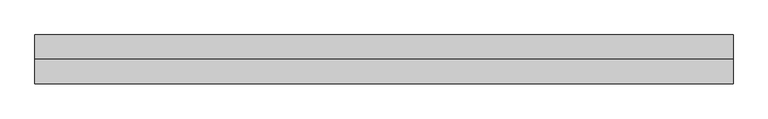
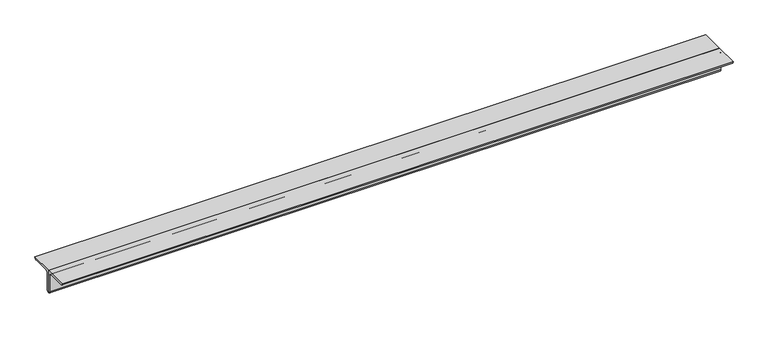
"""IFC4 building model written with IfcOpenShell, lengths in millimetres: member geometry, 0123_Steel Framing_2Ls-KSD3502 : H_SB_AR_S03_2Ls-130x130x12_HBR1."""

import ifcopenshell
import ifcopenshell.guid

model = None  # the IFC model being written
_history = None  # IfcOwnerHistory: only IFC2X3 demands one
_inside = {}  # id of a spatial element -> (the spatial element, [elements in it])
_under = {}  # id of a project, library or spatial element -> (it, [spatial elements below it])
_declared = {}  # id of a project -> (the project, [libraries it declares])
_typed = {}  # id of a type object -> (the type object, [elements of that type])
_made_of = {}  # id of a material, layer set ... -> (it, [elements and type objects made of it])


def new_model(schema):
    """Start an empty IFC model of exactly this schema.

    Asked for "IFC4X3", IfcOpenShell would pick the latest addendum, in which some entities
    have other attributes; the version numbers below select the first issue.
    IFC2X3 requires an IfcOwnerHistory on every rooted entity: one is made here for all.
    """
    global model, _history
    if schema == "IFC4X3":
        model = ifcopenshell.file(schema_version=(4, 3, 0, 0))
    else:
        model = ifcopenshell.file(schema=schema)
    _inside.clear()
    _under.clear()
    _declared.clear()
    _typed.clear()
    _made_of.clear()
    _history = None
    if model.schema == "IFC2X3":
        org = make("IfcOrganization", Name="unknown")
        user = make(
            "IfcPersonAndOrganization",
            ThePerson=make("IfcPerson", FamilyName="unknown"),
            TheOrganization=org,
        )
        app = make(
            "IfcApplication",
            ApplicationDeveloper=org,
            Version="unknown",
            ApplicationFullName="unknown",
            ApplicationIdentifier="unknown",
        )
        _history = make(
            "IfcOwnerHistory",
            OwningUser=user,
            OwningApplication=app,
            ChangeAction="ADDED",
            CreationDate=0,
        )
    return model


def make(cls, **values):
    """One entity of the class cls with the attributes given. An attribute that is None is left unset."""
    return model.create_entity(
        cls, **{name: value for name, value in values.items() if value is not None}
    )


def rooted(cls, **values):
    """An entity with a GlobalId (a new one), such as an element, a storey or a relation."""
    return make(cls, GlobalId=ifcopenshell.guid.new(), OwnerHistory=_history, **values)


def si_unit(unit_type, name, prefix=None):
    """IfcSIUnit, for example si_unit("LENGTHUNIT", "METRE", prefix="MILLI")."""
    return make("IfcSIUnit", UnitType=unit_type, Prefix=prefix, Name=name)


def assignment(units):
    """IfcUnitAssignment: the units of a project."""
    return None if units is None else make("IfcUnitAssignment", Units=units)


def point(xyz):
    """IfcCartesianPoint."""
    return None if xyz is None else make("IfcCartesianPoint", Coordinates=xyz)


def direction(xyz):
    """IfcDirection."""
    return None if xyz is None else make("IfcDirection", DirectionRatios=xyz)


def frame(location, z_axis=None, x_axis=None):
    """IfcAxis2Placement3D, a coordinate frame: its origin and axes. An axis left out is left unset."""
    return make(
        "IfcAxis2Placement3D",
        Location=point(location),
        Axis=direction(z_axis),
        RefDirection=direction(x_axis),
    )


def frame_2d(location, x_axis=None):
    """IfcAxis2Placement2D, a coordinate frame in the plane: its origin and x axis."""
    return make(
        "IfcAxis2Placement2D", Location=point(location), RefDirection=direction(x_axis)
    )


def origin():
    """The frame at (0, 0, 0) with its axes left unset."""
    return frame((0.0, 0.0, 0.0))


def place(relative_to, where):
    """IfcLocalPlacement: puts the frame where relative to a parent placement (None: the world)."""
    return make(
        "IfcLocalPlacement", PlacementRelTo=relative_to, RelativePlacement=where
    )


def context(
    kind, dimensions, precision=None, world=None, true_north=None, identifier=None
):
    """IfcGeometricRepresentationContext, for example the 3D "Model" context."""
    return make(
        "IfcGeometricRepresentationContext",
        ContextIdentifier=identifier,
        ContextType=kind,
        CoordinateSpaceDimension=dimensions,
        Precision=precision,
        WorldCoordinateSystem=world,
        TrueNorth=true_north,
    )


def project(units=None, contexts=None):
    """IfcProject with its units and contexts."""
    return rooted(
        "IfcProject",
        Name="project",
        RepresentationContexts=contexts,
        UnitsInContext=assignment(units),
    )


def spatial(cls, under=None, at=None, **own):
    """A site, building, storey or space (cls), placed at a placement, below another one or the project."""
    s = rooted(cls, ObjectPlacement=at, **own)
    if under is not None:
        _under.setdefault(under.id(), (under, []))[1].append(s)
    return s


def polyline(points):
    """IfcPolyline through the points."""
    return make("IfcPolyline", Points=[point(p) for p in points])


def circle_curve(where, radius):
    """IfcCircle in the frame where."""
    return make("IfcCircle", Position=where, Radius=radius)


def trimmed(basis, trim1, trim2, sense, master):
    """IfcTrimmedCurve: the piece of a basis curve between two trims."""
    return make(
        "IfcTrimmedCurve",
        BasisCurve=basis,
        Trim1=trim1,
        Trim2=trim2,
        SenseAgreement=sense,
        MasterRepresentation=master,
    )


def segment(curve, same_sense, transition):
    """IfcCompositeCurveSegment."""
    return make(
        "IfcCompositeCurveSegment",
        Transition=transition,
        SameSense=same_sense,
        ParentCurve=curve,
    )


def composite_curve(segments, self_intersect=None):
    """IfcCompositeCurve: segments joined end to end."""
    return make("IfcCompositeCurve", Segments=segments, SelfIntersect=self_intersect)


def outline(outer, holes=None, kind="AREA"):
    """IfcArbitraryClosedProfileDef: a profile drawn as a closed curve; with holes, ...WithVoids."""
    if holes is None:
        return make("IfcArbitraryClosedProfileDef", ProfileType=kind, OuterCurve=outer)
    return make(
        "IfcArbitraryProfileDefWithVoids",
        ProfileType=kind,
        OuterCurve=outer,
        InnerCurves=holes,
    )


def extrude(swept, where, along, depth):
    """IfcExtrudedAreaSolid: the profile swept, set in the frame where, extruded along a direction by depth."""
    return make(
        "IfcExtrudedAreaSolid",
        SweptArea=swept,
        Position=where,
        ExtrudedDirection=direction(along),
        Depth=depth,
    )


def shape(context_of_items, identifier, shape_type, items):
    """IfcShapeRepresentation: the items that make up one representation, for example the "Body"."""
    return make(
        "IfcShapeRepresentation",
        ContextOfItems=context_of_items,
        RepresentationIdentifier=identifier,
        RepresentationType=shape_type,
        Items=items,
    )


def source(mapping_origin, context_of_items, identifier, shape_type, items):
    """IfcRepresentationMap: a shape defined once, which mapped items show again and again."""
    return make(
        "IfcRepresentationMap",
        MappingOrigin=mapping_origin,
        MappedRepresentation=shape(context_of_items, identifier, shape_type, items),
    )


def transform(
    local_origin,
    x_axis=None,
    y_axis=None,
    z_axis=None,
    scale=None,
    scale2=None,
    scale3=None,
    uniform=True,
):
    """IfcCartesianTransformationOperator3D, or its non-uniform kind. x_axis, y_axis, z_axis: its Axis1, 2, 3."""
    if uniform:
        return make(
            "IfcCartesianTransformationOperator3D",
            Axis1=direction(x_axis),
            Axis2=direction(y_axis),
            LocalOrigin=point(local_origin),
            Scale=scale,
            Axis3=direction(z_axis),
        )
    return make(
        "IfcCartesianTransformationOperator3DnonUniform",
        Axis1=direction(x_axis),
        Axis2=direction(y_axis),
        LocalOrigin=point(local_origin),
        Scale=scale,
        Axis3=direction(z_axis),
        Scale2=scale2,
        Scale3=scale3,
    )


def mapped(mapping_source, mapping_target):
    """IfcMappedItem: shows the shape of a source again, moved by a transform."""
    return make(
        "IfcMappedItem", MappingSource=mapping_source, MappingTarget=mapping_target
    )


def made_of(thing, what):
    """Note that an element or type object is made of a material, layer set ...; save() writes the relation."""
    if what is not None:
        _made_of.setdefault(what.id(), (what, []))[1].append(thing)
    return thing


def element(
    cls,
    number,
    at=None,
    inside=None,
    cuts=None,
    type_object=None,
    material=None,
    context=None,
    identifier="Body",
    shape_type=None,
    held_by="IfcProductDefinitionShape",
    body=None,
    shapes=None,
    **own,
):
    """One element of the class cls, such as IfcWall. Its Tag is "e" and its number.

    at: its placement. inside: the storey or other place that contains it. cuts: it is an
    opening in that element (IfcRelVoidsElement). A single representation is given by context,
    identifier, shape_type and body (its items); several are given by shapes. held_by: the class
    of the entity that holds the representations. save() writes the other relations.
    """
    e = rooted(cls, Tag="e%d" % number, ObjectPlacement=at, **own)
    if body is not None:
        shapes = [shape(context, identifier, shape_type, body)]
    if shapes is not None:
        e.Representation = make(held_by, Representations=shapes)
    if inside is not None:
        _inside.setdefault(inside.id(), (inside, []))[1].append(e)
    if cuts is not None:
        rooted(
            "IfcRelVoidsElement", RelatingBuildingElement=cuts, RelatedOpeningElement=e
        )
    if type_object is not None:
        _typed.setdefault(type_object.id(), (type_object, []))[1].append(e)
    return made_of(e, material)


def aggregate(whole, parts):
    """IfcRelAggregates: a whole, such as a stair, and the parts it consists of."""
    return rooted("IfcRelAggregates", RelatingObject=whole, RelatedObjects=parts)


def save(model, path):
    """Write the relations noted so far, then the file.

    IfcRelAggregates (storeys below a building ...), IfcRelContainedInSpatialStructure (elements
    in a storey), IfcRelDefinesByType, IfcRelAssociatesMaterial and IfcRelDeclares: one each for
    every whole, place, type object, material and project.
    """
    for whole, parts in _under.values():
        aggregate(whole, parts)
    for where, things in _inside.values():
        rooted(
            "IfcRelContainedInSpatialStructure",
            RelatedElements=things,
            RelatingStructure=where,
        )
    for kind, things in _typed.values():
        rooted("IfcRelDefinesByType", RelatedObjects=things, RelatingType=kind)
    for what, things in _made_of.values():
        rooted("IfcRelAssociatesMaterial", RelatedObjects=things, RelatingMaterial=what)
    for by, libraries in _declared.values():
        rooted("IfcRelDeclares", RelatingContext=by, RelatedDefinitions=libraries)
    model.write(path)


def member_2dd2a1f8(model_context):
    return source(origin(), model_context, "Body", "SweptSolid", [
        extrude(outline(composite_curve([segment(polyline([(0.0, 36.4), (0.0, -93.6)]), True, "CONTINUOUS"), segment(trimmed(circle_curve(frame_2d((0.0, -81.6)), 12.0), [point((0.0, -93.6))], [point((-12.0, -81.6))], False, "CARTESIAN"), True, "CONTINUOUS"), segment(polyline([(-12.0, -81.6), (-12.0, 12.4)]), True, "CONTINUOUS"), segment(trimmed(circle_curve(frame_2d((-24.0, 12.4)), 12.0), [point((-12.0, 12.4))], [point((-24.0, 24.4))], True, "CARTESIAN"), True, "CONTINUOUS"), segment(polyline([(-24.0, 24.4), (-118.0, 24.4)]), True, "CONTINUOUS"), segment(trimmed(circle_curve(frame_2d((-118.0, 36.4)), 12.0), [point((-118.0, 24.4))], [point((-130.0, 36.4))], False, "CARTESIAN"), True, "CONTINUOUS"), segment(polyline([(-130.0, 36.4), (0.0, 36.4)]), True, "CONTINUOUS")], self_intersect=False)), frame((-1830.7666695, 0.0, 0.0), z_axis=(1.0, 0.0, 0.0), x_axis=(0.0, 1.0, 0.0)), (0.0, 0.0, 1.0), 3701.6272171),
        extrude(outline(composite_curve([segment(polyline([(0.0, 36.4), (130.0, 36.4)]), True, "CONTINUOUS"), segment(trimmed(circle_curve(frame_2d((118.0, 36.4)), 12.0), [point((130.0, 36.4))], [point((118.0, 24.4))], False, "CARTESIAN"), True, "CONTINUOUS"), segment(polyline([(118.0, 24.4), (24.0, 24.4)]), True, "CONTINUOUS"), segment(trimmed(circle_curve(frame_2d((24.0, 12.4)), 12.0), [point((24.0, 24.4))], [point((12.0, 12.4))], True, "CARTESIAN"), True, "CONTINUOUS"), segment(polyline([(12.0, 12.4), (12.0, -81.6)]), True, "CONTINUOUS"), segment(trimmed(circle_curve(frame_2d((0.0, -81.6)), 12.0), [point((12.0, -81.6))], [point((0.0, -93.6))], False, "CARTESIAN"), True, "CONTINUOUS"), segment(polyline([(0.0, -93.6), (0.0, 36.4)]), True, "CONTINUOUS")], self_intersect=False)), frame((-1830.7666695, 0.0, 0.0), z_axis=(1.0, 0.0, 0.0), x_axis=(0.0, 1.0, 0.0)), (0.0, 0.0, 1.0), 3701.6272171),
    ])


if __name__ == "__main__":
    model = new_model("IFC4")
    model_context = context("Model", 3, world=origin())
    ifc_project = project(units=[si_unit("LENGTHUNIT", "METRE", prefix="MILLI")], contexts=[model_context])
    site = spatial("IfcSite", under=ifc_project)
    building = spatial("IfcBuilding", under=site)
    placement = place(None, origin())
    member_shape = member_2dd2a1f8(model_context)
    element("IfcMember", 1, ObjectType="0123_Steel Framing_2Ls-KSD3502 : H_SB_AR_S03_2Ls-130x130x12_HBR1", at=placement, inside=building, context=model_context, shape_type="MappedRepresentation", body=[
        mapped(member_shape, transform((0.0, 0.0, 0.0), x_axis=(1.0, 0.0, 0.0), y_axis=(0.0, 1.0, 0.0), z_axis=(0.0, 0.0, 1.0))),
    ])
    save(model, "model.ifc")

# Revit data of these elements
# Type "0123_Steel Framing_2Ls-KSD3502 : H_SB_AR_S03_2Ls-130x130x12_HBR1"
#   Assembly Code = "B10"
#   Legs = "SLBB"
#   W = 8.97
#   Perimeter = 1.04 m²/m
#   Nominal Weight = 46.80 kgf/m
#   Length [instance default] = 1000 mm
#   Space = 0 mm
#   b = 130 mm
#   d = 130 mm
#   t = 12 mm
#   y = 36.4 mm
#   A = 0.005952 m²
#   Structural Material [instance default] = Steel ASTM A36
# Element 1 (IfcMember, "0123_Steel Framing_2Ls-KSD3502 : H_SB_AR_S03_2Ls-130x130x12_HBR1")
#   Structural Material = Steel, 45-345
#   Materials on its faces: "Steel, 45-345"
# Materials
#   "Steel ASTM A36": class "Metal", colour RGB 199 199 199, transparency 0, Description = "Structural steel, ASTM A36 Grade B, mill finish", Cost = 0
#   "Steel, 45-345": class "Metal", colour RGB 189 187 185, transparency 0, Description = "Steel 345 MPa", Cost = 0
